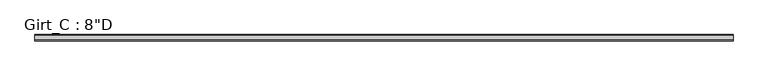
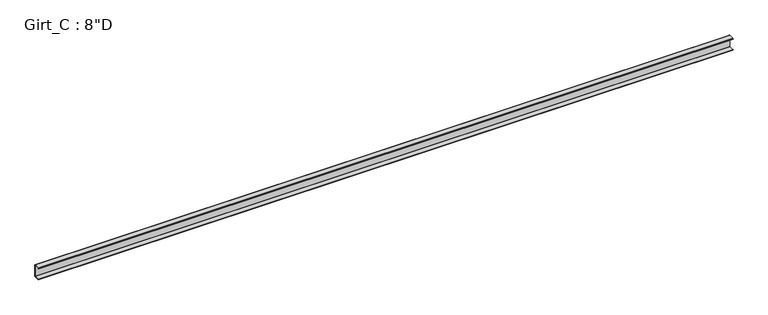
"""IFC4 building model written with IfcOpenShell, lengths in millimetres: beam geometry."""

from ifc_helpers import new_model, si_unit, point, frame, frame_2d, origin, place, context, project, spatial, polyline, circle_curve, trimmed, segment, composite_curve, outline, extrude, source, transform, mapped, element, save


def beam_22ebce67(model_context):
    return source(origin(), model_context, "Body", "SweptSolid", [
        extrude(outline(composite_curve([segment(polyline([(-87.5109375, 101.6), (-3.3734375, 101.6)]), True, "CONTINUOUS"), segment(trimmed(circle_curve(frame_2d((-3.3734375, 96.8375)), 4.7625), [point((-3.3734375, 101.6))], [point((1.3890625, 96.8375))], False, "CARTESIAN"), True, "CONTINUOUS"), segment(polyline([(1.3890625, 96.8375), (1.3890625, -96.8375)]), True, "CONTINUOUS"), segment(trimmed(circle_curve(frame_2d((-3.3734375, -96.8375)), 4.7625), [point((1.3890625, -96.8375))], [point((-3.3734375, -101.6))], False, "CARTESIAN"), True, "CONTINUOUS"), segment(polyline([(-3.3734375, -101.6), (-87.5109375, -101.6), (-99.7792647, -86.979177), (-97.6510975, -85.1934327), (-86.2154765, -98.821875), (-3.2694106, -98.821875)]), True, "CONTINUOUS"), segment(trimmed(circle_curve(frame_2d((-3.3748024, -96.8389339)), 1.9857399), [point((-3.2694106, -98.821875))], [point((-1.3890625, -96.8389339))], True, "CARTESIAN"), True, "CONTINUOUS"), segment(polyline([(-1.3890625, -96.8389339), (-1.3890625, 96.8381931)]), True, "CONTINUOUS"), segment(trimmed(circle_curve(frame_2d((-3.3741066, 96.8381931)), 1.9850441), [point((-1.3890625, 96.8381931))], [point((-3.3005807, 98.821875))], True, "CARTESIAN"), True, "CONTINUOUS"), segment(polyline([(-3.3005807, 98.821875), (-86.2154765, 98.821875), (-97.6278742, 85.221109), (-99.7560415, 87.0068534), (-87.5109375, 101.6)]), True, "CONTINUOUS")], self_intersect=False)), frame((-5553.075, 0.0, 0.0), z_axis=(1.0, 0.0, 0.0), x_axis=(0.0, 1.0, 0.0)), (0.0, 0.0, 1.0), 11106.15),
    ])


if __name__ == "__main__":
    model = new_model("IFC4")
    model_context = context("Model", 3, world=origin())
    ifc_project = project(units=[si_unit("LENGTHUNIT", "METRE", prefix="MILLI")], contexts=[model_context])
    site = spatial("IfcSite", under=ifc_project)
    building = spatial("IfcBuilding", under=site)
    placement = place(None, origin())
    beam_shape = beam_22ebce67(model_context)
    element("IfcBeam", 1, ObjectType="Girt_C : 8\"D", at=placement, inside=building, context=model_context, shape_type="MappedRepresentation", body=[
        mapped(beam_shape, transform((0.0, 0.0, 0.0), x_axis=(1.0, 0.0, 0.0), y_axis=(0.0, 1.0, 0.0), z_axis=(0.0, 0.0, 1.0))),
    ])
    save(model, "model.ifc")

# Revit data of these elements
# Type "Girt_C : 8\"D"
#   half leg = 0' - 1 3/4"
#   Web_Thickness = 0' - 0 7/64"
#   Length [instance default] = 10' - 0"
#   Leg_1 = 0' - 3 1/2"
#   Height = 0' - 8"
#   Structural Material [instance default] = none
# Element 1 (IfcBeam, "Girt_C : 8\"D")
#   Structural Material = CEE' SECTION (8.0x3.5C - SEE STRUCT. DWGS)
#   Materials on its faces: "CEE' SECTION (8.0x3.5C - SEE STRUCT. DWGS)"
# Materials
#   "CEE' SECTION (8.0x3.5C - SEE STRUCT. DWGS)": class "Metal", colour RGB 137 146 153, transparency 0, Description = "Steel, mill finish", Cost = 0
